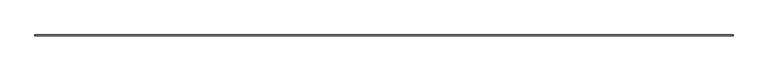
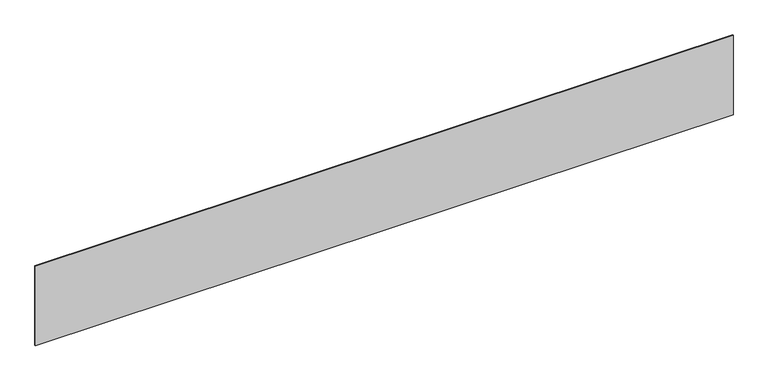
"""IFC4 building model written with IfcOpenShell, lengths in millimetres: proxy geometry, Inner panel:Inner panel:1:Inner panel:1 : Inner panel:Inner panel:300324:300043:Inner panel:1:Inner panel:1 : Inner panel:Inner panel:300324:300043 : Inner panel:Inner panel:1:Inner panel:1 : Inner panel:Inner panel:300324:300043:12 : Inner panel:Inner panel:1:Inner panel:1 : Inner panel:Inner panel:300324:300043:Inner panel:1:Inner panel:1 : Inner panel:Inner panel:300324:300043 : Inner panel:Inner panel:1:Inner panel:1 : Inner panel:Inner panel:300324:300043:300031."""

import ifcopenshell
import ifcopenshell.guid

model = None  # the IFC model being written
_history = None  # IfcOwnerHistory: only IFC2X3 demands one
_inside = {}  # id of a spatial element -> (the spatial element, [elements in it])
_under = {}  # id of a project, library or spatial element -> (it, [spatial elements below it])
_declared = {}  # id of a project -> (the project, [libraries it declares])
_typed = {}  # id of a type object -> (the type object, [elements of that type])
_made_of = {}  # id of a material, layer set ... -> (it, [elements and type objects made of it])


def new_model(schema):
    """Start an empty IFC model of exactly this schema.

    Asked for "IFC4X3", IfcOpenShell would pick the latest addendum, in which some entities
    have other attributes; the version numbers below select the first issue.
    IFC2X3 requires an IfcOwnerHistory on every rooted entity: one is made here for all.
    """
    global model, _history
    if schema == "IFC4X3":
        model = ifcopenshell.file(schema_version=(4, 3, 0, 0))
    else:
        model = ifcopenshell.file(schema=schema)
    _inside.clear()
    _under.clear()
    _declared.clear()
    _typed.clear()
    _made_of.clear()
    _history = None
    if model.schema == "IFC2X3":
        org = make("IfcOrganization", Name="unknown")
        user = make(
            "IfcPersonAndOrganization",
            ThePerson=make("IfcPerson", FamilyName="unknown"),
            TheOrganization=org,
        )
        app = make(
            "IfcApplication",
            ApplicationDeveloper=org,
            Version="unknown",
            ApplicationFullName="unknown",
            ApplicationIdentifier="unknown",
        )
        _history = make(
            "IfcOwnerHistory",
            OwningUser=user,
            OwningApplication=app,
            ChangeAction="ADDED",
            CreationDate=0,
        )
    return model


def make(cls, **values):
    """One entity of the class cls with the attributes given. An attribute that is None is left unset."""
    return model.create_entity(
        cls, **{name: value for name, value in values.items() if value is not None}
    )


def rooted(cls, **values):
    """An entity with a GlobalId (a new one), such as an element, a storey or a relation."""
    return make(cls, GlobalId=ifcopenshell.guid.new(), OwnerHistory=_history, **values)


def si_unit(unit_type, name, prefix=None):
    """IfcSIUnit, for example si_unit("LENGTHUNIT", "METRE", prefix="MILLI")."""
    return make("IfcSIUnit", UnitType=unit_type, Prefix=prefix, Name=name)


def assignment(units):
    """IfcUnitAssignment: the units of a project."""
    return None if units is None else make("IfcUnitAssignment", Units=units)


def point(xyz):
    """IfcCartesianPoint."""
    return None if xyz is None else make("IfcCartesianPoint", Coordinates=xyz)


def direction(xyz):
    """IfcDirection."""
    return None if xyz is None else make("IfcDirection", DirectionRatios=xyz)


def frame(location, z_axis=None, x_axis=None):
    """IfcAxis2Placement3D, a coordinate frame: its origin and axes. An axis left out is left unset."""
    return make(
        "IfcAxis2Placement3D",
        Location=point(location),
        Axis=direction(z_axis),
        RefDirection=direction(x_axis),
    )


def origin():
    """The frame at (0, 0, 0) with its axes left unset."""
    return frame((0.0, 0.0, 0.0))


def place(relative_to, where):
    """IfcLocalPlacement: puts the frame where relative to a parent placement (None: the world)."""
    return make(
        "IfcLocalPlacement", PlacementRelTo=relative_to, RelativePlacement=where
    )


def context(
    kind, dimensions, precision=None, world=None, true_north=None, identifier=None
):
    """IfcGeometricRepresentationContext, for example the 3D "Model" context."""
    return make(
        "IfcGeometricRepresentationContext",
        ContextIdentifier=identifier,
        ContextType=kind,
        CoordinateSpaceDimension=dimensions,
        Precision=precision,
        WorldCoordinateSystem=world,
        TrueNorth=true_north,
    )


def project(units=None, contexts=None):
    """IfcProject with its units and contexts."""
    return rooted(
        "IfcProject",
        Name="project",
        RepresentationContexts=contexts,
        UnitsInContext=assignment(units),
    )


def spatial(cls, under=None, at=None, **own):
    """A site, building, storey or space (cls), placed at a placement, below another one or the project."""
    s = rooted(cls, ObjectPlacement=at, **own)
    if under is not None:
        _under.setdefault(under.id(), (under, []))[1].append(s)
    return s


def polyline(points):
    """IfcPolyline through the points."""
    return make("IfcPolyline", Points=[point(p) for p in points])


def outline(outer, holes=None, kind="AREA"):
    """IfcArbitraryClosedProfileDef: a profile drawn as a closed curve; with holes, ...WithVoids."""
    if holes is None:
        return make("IfcArbitraryClosedProfileDef", ProfileType=kind, OuterCurve=outer)
    return make(
        "IfcArbitraryProfileDefWithVoids",
        ProfileType=kind,
        OuterCurve=outer,
        InnerCurves=holes,
    )


def extrude(swept, where, along, depth):
    """IfcExtrudedAreaSolid: the profile swept, set in the frame where, extruded along a direction by depth."""
    return make(
        "IfcExtrudedAreaSolid",
        SweptArea=swept,
        Position=where,
        ExtrudedDirection=direction(along),
        Depth=depth,
    )


def shape(context_of_items, identifier, shape_type, items):
    """IfcShapeRepresentation: the items that make up one representation, for example the "Body"."""
    return make(
        "IfcShapeRepresentation",
        ContextOfItems=context_of_items,
        RepresentationIdentifier=identifier,
        RepresentationType=shape_type,
        Items=items,
    )


def source(mapping_origin, context_of_items, identifier, shape_type, items):
    """IfcRepresentationMap: a shape defined once, which mapped items show again and again."""
    return make(
        "IfcRepresentationMap",
        MappingOrigin=mapping_origin,
        MappedRepresentation=shape(context_of_items, identifier, shape_type, items),
    )


def transform(
    local_origin,
    x_axis=None,
    y_axis=None,
    z_axis=None,
    scale=None,
    scale2=None,
    scale3=None,
    uniform=True,
):
    """IfcCartesianTransformationOperator3D, or its non-uniform kind. x_axis, y_axis, z_axis: its Axis1, 2, 3."""
    if uniform:
        return make(
            "IfcCartesianTransformationOperator3D",
            Axis1=direction(x_axis),
            Axis2=direction(y_axis),
            LocalOrigin=point(local_origin),
            Scale=scale,
            Axis3=direction(z_axis),
        )
    return make(
        "IfcCartesianTransformationOperator3DnonUniform",
        Axis1=direction(x_axis),
        Axis2=direction(y_axis),
        LocalOrigin=point(local_origin),
        Scale=scale,
        Axis3=direction(z_axis),
        Scale2=scale2,
        Scale3=scale3,
    )


def mapped(mapping_source, mapping_target):
    """IfcMappedItem: shows the shape of a source again, moved by a transform."""
    return make(
        "IfcMappedItem", MappingSource=mapping_source, MappingTarget=mapping_target
    )


def made_of(thing, what):
    """Note that an element or type object is made of a material, layer set ...; save() writes the relation."""
    if what is not None:
        _made_of.setdefault(what.id(), (what, []))[1].append(thing)
    return thing


def element(
    cls,
    number,
    at=None,
    inside=None,
    cuts=None,
    type_object=None,
    material=None,
    context=None,
    identifier="Body",
    shape_type=None,
    held_by="IfcProductDefinitionShape",
    body=None,
    shapes=None,
    **own,
):
    """One element of the class cls, such as IfcWall. Its Tag is "e" and its number.

    at: its placement. inside: the storey or other place that contains it. cuts: it is an
    opening in that element (IfcRelVoidsElement). A single representation is given by context,
    identifier, shape_type and body (its items); several are given by shapes. held_by: the class
    of the entity that holds the representations. save() writes the other relations.
    """
    e = rooted(cls, Tag="e%d" % number, ObjectPlacement=at, **own)
    if body is not None:
        shapes = [shape(context, identifier, shape_type, body)]
    if shapes is not None:
        e.Representation = make(held_by, Representations=shapes)
    if inside is not None:
        _inside.setdefault(inside.id(), (inside, []))[1].append(e)
    if cuts is not None:
        rooted(
            "IfcRelVoidsElement", RelatingBuildingElement=cuts, RelatedOpeningElement=e
        )
    if type_object is not None:
        _typed.setdefault(type_object.id(), (type_object, []))[1].append(e)
    return made_of(e, material)


def aggregate(whole, parts):
    """IfcRelAggregates: a whole, such as a stair, and the parts it consists of."""
    return rooted("IfcRelAggregates", RelatingObject=whole, RelatedObjects=parts)


def save(model, path):
    """Write the relations noted so far, then the file.

    IfcRelAggregates (storeys below a building ...), IfcRelContainedInSpatialStructure (elements
    in a storey), IfcRelDefinesByType, IfcRelAssociatesMaterial and IfcRelDeclares: one each for
    every whole, place, type object, material and project.
    """
    for whole, parts in _under.values():
        aggregate(whole, parts)
    for where, things in _inside.values():
        rooted(
            "IfcRelContainedInSpatialStructure",
            RelatedElements=things,
            RelatingStructure=where,
        )
    for kind, things in _typed.values():
        rooted("IfcRelDefinesByType", RelatedObjects=things, RelatingType=kind)
    for what, things in _made_of.values():
        rooted("IfcRelAssociatesMaterial", RelatedObjects=things, RelatingMaterial=what)
    for by, libraries in _declared.values():
        rooted("IfcRelDeclares", RelatingContext=by, RelatedDefinitions=libraries)
    model.write(path)


def generic_models_7a503c72(model_context):
    return source(origin(), model_context, "Body", "SweptSolid", [
        extrude(outline(polyline([(560299.271048, -579051.4913841), (570446.2867239, -579051.4913841), (570446.2867239, -579064.1913841), (560299.271048, -579064.1913841), (560299.271048, -579051.4913841)])), frame((0.0, 0.0, 4927.6), z_axis=(0.0, 0.0, 1.0), x_axis=(1.0, 0.0, 0.0)), (0.0, 0.0, 1.0), 1219.2),
    ])


if __name__ == "__main__":
    model = new_model("IFC4")
    model_context = context("Model", 3, world=origin())
    ifc_project = project(units=[si_unit("LENGTHUNIT", "METRE", prefix="MILLI")], contexts=[model_context])
    site = spatial("IfcSite", under=ifc_project)
    building = spatial("IfcBuilding", under=site)
    placement = place(None, origin())
    generic_models_shape = generic_models_7a503c72(model_context)
    element("IfcBuildingElementProxy", 1, Name="Inner panel:Inner panel:1:Inner panel:1 : Inner panel:Inner panel:300324:300043:Inner panel:1:Inner panel:1 : Inner panel:Inner panel:300324:300043 : Inner panel:Inner panel:1:Inner panel:1 : Inner panel:Inner panel:300324:300043:12 : Inner panel:Inner panel:1:Inner panel:1 : Inner panel:Inner panel:300324:300043:Inner panel:1:Inner panel:1 : Inner panel:Inner panel:300324:300043 : Inner panel:Inner panel:1:Inner panel:1 : Inner panel:Inner panel:300324:300043:300031", ObjectType="Inner panel:Inner panel:1:Inner panel:1 : Inner panel:Inner panel:300324:300043:Inner panel:1:Inner panel:1 : Inner panel:Inner panel:300324:300043 : Inner panel:Inner panel:1:Inner panel:1 : Inner panel:Inner panel:300324:300043:12 : Inner panel:Inner panel:1:Inner panel:1 : Inner panel:Inner panel:300324:300043:Inner panel:1:Inner panel:1 : Inner panel:Inner panel:300324:300043 : Inner panel:Inner panel:1:Inner panel:1 : Inner panel:Inner panel:300324:300043:300031", at=placement, inside=building, context=model_context, shape_type="MappedRepresentation", body=[
        mapped(generic_models_shape, transform((0.0, 0.0, 0.0), x_axis=(1.0, 0.0, 0.0), y_axis=(0.0, 1.0, 0.0), z_axis=(0.0, 0.0, 1.0))),
    ])
    save(model, "model.ifc")

# Revit data of these elements
# Type "Inner panel:Inner panel:1:Inner panel:1 : Inner panel:Inner panel:300324:300043:Inner panel:1:Inner panel:1 : Inner panel:Inner panel:300324:300043 : Inner panel:Inner panel:1:Inner panel:1 : Inner panel:Inner panel:300324:300043:12 : Inner panel:Inner panel:1:Inner panel:1 : Inner panel:Inner panel:300324:300043:Inner panel:1:Inner panel:1 : Inner panel:Inner panel:300324:300043 : Inner panel:Inner panel:1:Inner panel:1 : Inner panel:Inner panel:300324:300043:300031"
#   NameOverride = "Inner panel:Inner panel:1:Inner panel:1 : Inner panel:Inner panel:300324:300043:Inner panel:1:Inner panel:1 : Inner panel:Inner panel:300324:300043 : Inner panel:Inner panel:1:Inner panel:1 : Inner panel:Inner panel:300324:300043:300031"
#   ObjectTypeOverride = "Inner panel:1:Inner panel:1 : Inner panel:Inner panel:300324:300043 : Inner panel:Inner panel:1:Inner panel:1 : Inner panel:Inner panel:300324:300043"
#   Reference = "Inner panel"
#   Tag = "300031"
# Element 1 (IfcBuildingElementProxy, "Inner panel:Inner panel:1:Inner panel:1 : Inner panel:Inner panel:300324:300043:Inner panel:1:Inner panel:1 : Inner panel:Inner panel:300324:300043 : Inner panel:Inner panel:1:Inner panel:1 : Inner panel:Inner panel:300324:300043:12 : Inner panel:Inner panel:1:Inner panel:1 : Inner panel:Inner panel:300324:300043:Inner panel:1:Inner panel:1 : Inner panel:Inner panel:300324:300043 : Inner panel:Inner panel:1:Inner panel:1 : Inner panel:Inner panel:300324:300043:300031")
#   Materials on its faces: "1/2\" EXTERIOR GRADE FIRE RETARDANT CDX PLYWOOD"
# Materials
#   "1/2\" EXTERIOR GRADE FIRE RETARDANT CDX PLYWOOD": class "Unassigned", colour RGB 196 177 123, transparency 0, Cost = 0
